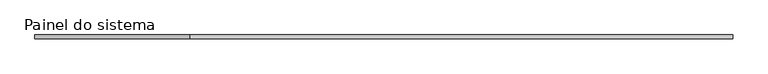
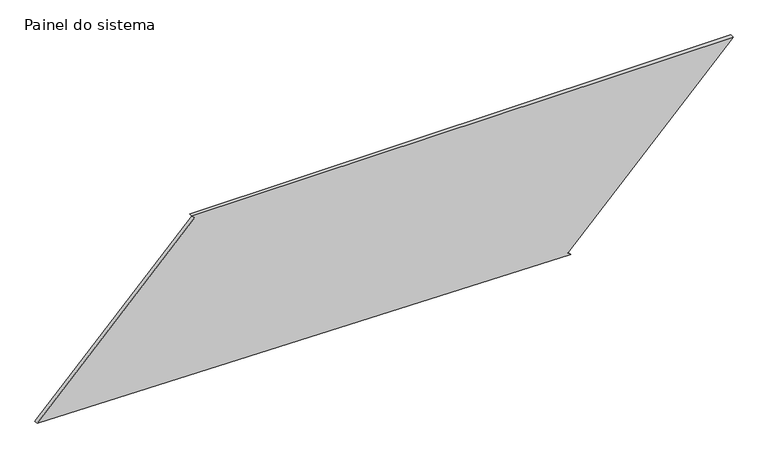
"""IFC4 building model written with IfcOpenShell, lengths in millimetres: plate geometry, Painel do sistema : Envidraçado."""

from ifc_helpers import new_model, si_unit, frame, origin, place, context, project, spatial, polyline, outline, extrude, source, transform, mapped, element, save


def painel_do_sistema_bfc6f6d1(model_context):
    return source(origin(), model_context, "Body", "SweptSolid", [
        extrude(outline(polyline([(0.0, 1215.3142487), (17.3932625, 1197.356676), (1135.3725319, 2280.2038546), (1135.3725319, -1266.5295737), (1117.9792693, -1248.572001), (52.8769643, -2280.2038546), (0.0, 1215.3142487)])), frame((0.0, 24.5, 0.0), z_axis=(0.0, 1.0, 0.0), x_axis=(0.0, 0.0, 1.0)), (0.0, 0.0, 1.0), 25.0),
    ])


if __name__ == "__main__":
    model = new_model("IFC4")
    model_context = context("Model", 3, world=origin())
    ifc_project = project(units=[si_unit("LENGTHUNIT", "METRE", prefix="MILLI")], contexts=[model_context])
    site = spatial("IfcSite", under=ifc_project)
    building = spatial("IfcBuilding", under=site)
    placement = place(None, origin())
    painel_do_sistema_shape = painel_do_sistema_bfc6f6d1(model_context)
    element("IfcPlate", 1, ObjectType="Painel do sistema : Envidraçado", at=placement, inside=building, context=model_context, shape_type="MappedRepresentation", body=[
        mapped(painel_do_sistema_shape, transform((0.0, 0.0, 0.0), x_axis=(1.0, 0.0, 0.0), y_axis=(0.0, 1.0, 0.0), z_axis=(0.0, 0.0, 1.0))),
    ])
    save(model, "model.ifc")

# Revit data of these elements
# Type "Painel do sistema : Envidraçado"
#   Construction Type Id = "GSP4R"
#   Analytic Construction = "Vidraça única Pilkington 1/8 pol"
#   Visual Light Transmittance = 0.9
#   Solar Heat Gain Coefficient = 0.86
#   Heat Transfer Coefficient (U) = 6.7069 W/(m²·K)
# Element 1 (IfcPlate, "Painel do sistema : Envidraçado")
#   Materials on its faces: "Vidro"
# Materials
#   "Vidro": class "Vidro", colour RGB 0 128 192, transparency 0.9, Description = "Vidro de sílica", Cost = 0
